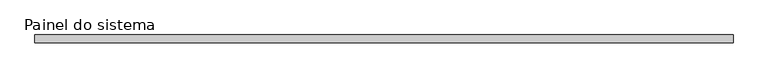
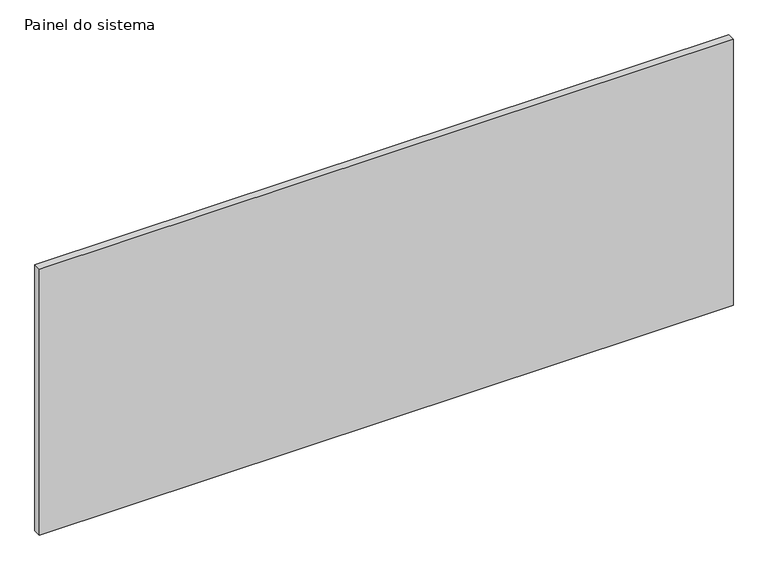
"""IFC4 building model written with IfcOpenShell, lengths in millimetres: plate geometry, Painel do sistema : Envidraçado."""

from ifc_helpers import new_model, si_unit, origin, origin_with_axes, place, context, project, spatial, polyline, outline, extrude, source, transform, mapped, element, save


def painel_do_sistema_da667d39(model_context):
    return source(origin(), model_context, "Body", "SweptSolid", [
        extrude(outline(polyline([(1110.3819696, -49.5), (-1110.3819696, -49.5), (-1110.3819696, -24.5), (1110.3819696, -24.5), (1110.3819696, -49.5)])), origin_with_axes(), (0.0, 0.0, 1.0), 900.0),
    ])


if __name__ == "__main__":
    model = new_model("IFC4")
    model_context = context("Model", 3, world=origin())
    ifc_project = project(units=[si_unit("LENGTHUNIT", "METRE", prefix="MILLI")], contexts=[model_context])
    site = spatial("IfcSite", under=ifc_project)
    building = spatial("IfcBuilding", under=site)
    placement = place(None, origin())
    painel_do_sistema_shape = painel_do_sistema_da667d39(model_context)
    element("IfcPlate", 1, ObjectType="Painel do sistema : Envidraçado", at=placement, inside=building, context=model_context, shape_type="MappedRepresentation", body=[
        mapped(painel_do_sistema_shape, transform((0.0, 0.0, 0.0), x_axis=(1.0, 0.0, 0.0), y_axis=(0.0, 1.0, 0.0), z_axis=(0.0, 0.0, 1.0))),
    ])
    save(model, "model.ifc")

# Revit data of these elements
# Type "Painel do sistema : Envidraçado"
#   Construction Type Id = "GSP4R"
#   Analytic Construction = "Vidraça única Pilkington 1/8 pol"
#   Visual Light Transmittance = 0.9
#   Solar Heat Gain Coefficient = 0.86
#   Heat Transfer Coefficient (U) = 6.7069 W/(m²·K)
# Element 1 (IfcPlate, "Painel do sistema : Envidraçado")
#   Materials on its faces: "Vidro"
# Materials
#   "Vidro": class "Vidro", colour RGB 0 128 192, transparency 0.9, Description = "Vidro de sílica", Cost = 0
